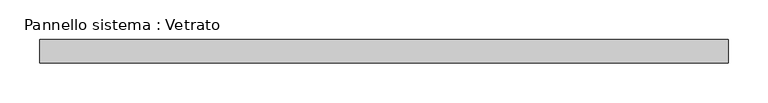
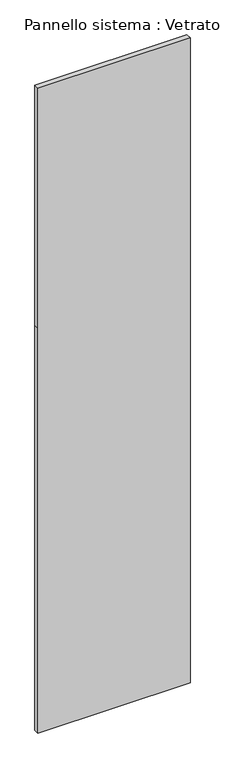
"""IFC4 building model written with IfcOpenShell, lengths in millimetres: plate geometry, Pannello sistema : Vetrato."""

from ifc_helpers import new_model, si_unit, frame, origin, place, context, project, spatial, polyline, outline, extrude, source, transform, mapped, element, save


def pannello_sistema_vetrato_69173132(model_context):
    return source(origin(), model_context, "Body", "SweptSolid", [
        extrude(outline(polyline([(0.0, -435.0), (0.0, 435.0), (2450.0, 435.0), (3900.0, 435.0), (3900.0, -435.0), (2450.0, -435.0), (0.0, -435.0)])), frame((0.0, -15.0, 0.0), z_axis=(0.0, 1.0, 0.0), x_axis=(0.0, 0.0, 1.0)), (0.0, 0.0, 1.0), 30.0),
    ])


if __name__ == "__main__":
    model = new_model("IFC4")
    model_context = context("Model", 3, world=origin())
    ifc_project = project(units=[si_unit("LENGTHUNIT", "METRE", prefix="MILLI")], contexts=[model_context])
    site = spatial("IfcSite", under=ifc_project)
    building = spatial("IfcBuilding", under=site)
    placement = place(None, origin())
    pannello_sistema_vetrato_shape = pannello_sistema_vetrato_69173132(model_context)
    element("IfcPlate", 1, ObjectType="Pannello sistema : Vetrato", at=placement, inside=building, context=model_context, shape_type="MappedRepresentation", body=[
        mapped(pannello_sistema_vetrato_shape, transform((0.0, 0.0, 0.0), x_axis=(1.0, 0.0, 0.0), y_axis=(0.0, 1.0, 0.0), z_axis=(0.0, 0.0, 1.0))),
    ])
    save(model, "model.ifc")

# Revit data of these elements
# Type "Pannello sistema : Vetrato"
#   Construction Type Id = "GSP4R"
#   Analytic Construction = "Vetrata singola Pilkington 1/8 in"
#   Visual Light Transmittance = 0.9
#   Solar Heat Gain Coefficient = 0.86
#   Heat Transfer Coefficient (U) = 6.7069 W/(m²·K)
# Element 1 (IfcPlate, "Pannello sistema : Vetrato")
#   Materials on its faces: "Default - Vetro"
# Materials
#   "Default - Vetro": class "Vetro", colour RGB 208 208 208, transparency 0.7, Cost = 0
